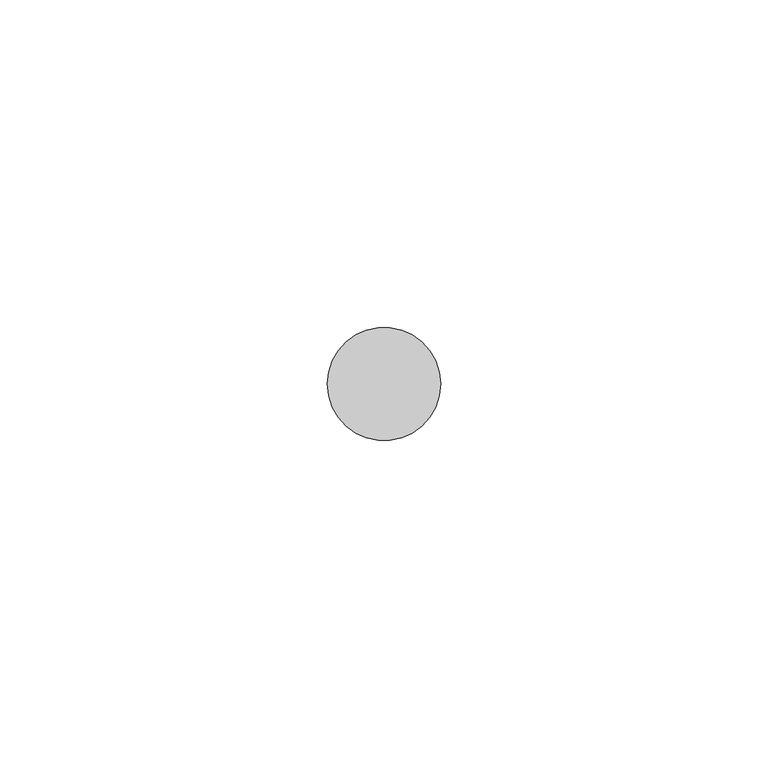
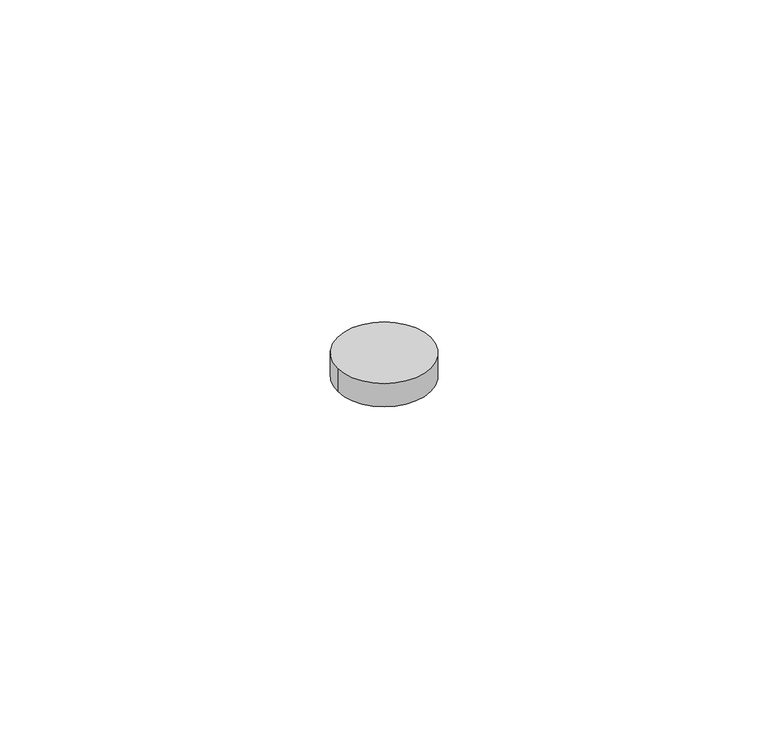
"""IFC4 building model written with IfcOpenShell, lengths in millimetres: proxy geometry, Hinge Pin Keeper5 : Hinge Pin Keeper."""

from ifc_helpers import new_model, si_unit, point, frame, frame_2d, origin, place, context, project, spatial, circle_curve, trimmed, segment, composite_curve, outline, extrude, source, transform, mapped, element, save


def generic_models_87e8abe8(model_context):
    return source(origin(), model_context, "Body", "SweptSolid", [
        extrude(outline(composite_curve([segment(trimmed(circle_curve(frame_2d((587319.1320739, -533984.6777841)), 8.6534625), [point((587310.4786114, -533984.6777841))], [point((587327.7855364, -533984.6777841))], False, "CARTESIAN"), True, "CONTINUOUS"), segment(trimmed(circle_curve(frame_2d((587319.1320739, -533984.6777841)), 8.6534625), [point((587327.7855364, -533984.6777841))], [point((587310.4786114, -533984.6777841))], False, "CARTESIAN"), True, "CONTINUOUS")], self_intersect=False)), frame((0.0, 0.0, 1271.7859375), z_axis=(0.0, 0.0, 1.0), x_axis=(1.0, 0.0, 0.0)), (0.0, 0.0, 1.0), 4.5640625),
    ])


if __name__ == "__main__":
    model = new_model("IFC4")
    model_context = context("Model", 3, world=origin())
    ifc_project = project(units=[si_unit("LENGTHUNIT", "METRE", prefix="MILLI")], contexts=[model_context])
    site = spatial("IfcSite", under=ifc_project)
    building = spatial("IfcBuilding", under=site)
    placement = place(None, origin())
    generic_models_shape = generic_models_87e8abe8(model_context)
    element("IfcBuildingElementProxy", 1, Name="Hinge Pin Keeper5 : Hinge Pin Keeper", ObjectType="Hinge Pin Keeper5 : Hinge Pin Keeper", at=placement, inside=building, context=model_context, shape_type="MappedRepresentation", body=[
        mapped(generic_models_shape, transform((0.0, 0.0, 0.0), x_axis=(1.0, 0.0, 0.0), y_axis=(0.0, 1.0, 0.0), z_axis=(0.0, 0.0, 1.0))),
    ])
    save(model, "model.ifc")

# Revit data of these elements
# Element 1 (IfcBuildingElementProxy, "Hinge Pin Keeper5 : Hinge Pin Keeper")
#   Materials on its faces: "6\"X6\" WELD-ON STL BUTT HINGE"
# Materials
#   "6\"X6\" WELD-ON STL BUTT HINGE": class "Metal", colour RGB 189 187 185, transparency 0, Description = "Carbon steel", Cost = 0
